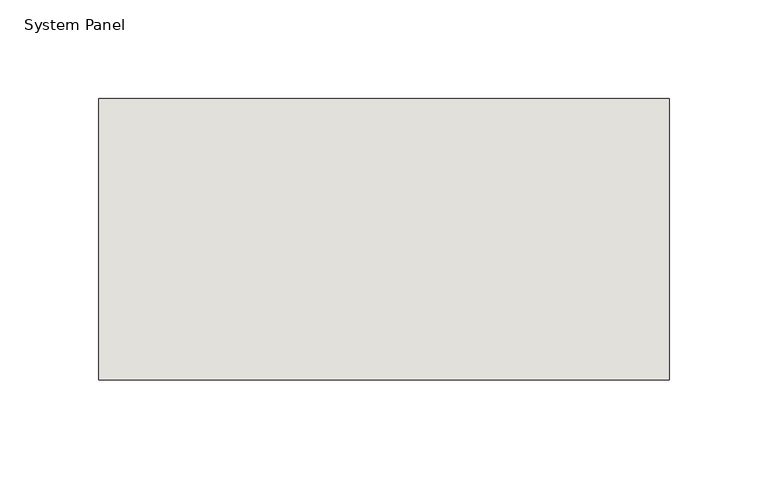
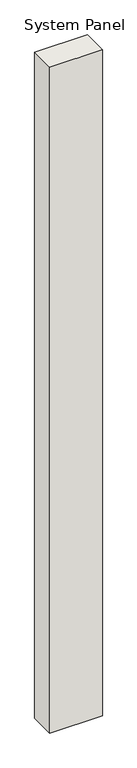
"""IFC4 building model written with IfcOpenShell, lengths in millimetres: wall geometry, System Panel : NLRS_21_CWP_hsb-vulling minerale wol 142 _gen_rsf."""

from ifc_helpers import new_model, si_unit, origin, origin_with_axes, place, context, project, spatial, polyline, outline, extrude, source, transform, mapped, element, save


def system_panel_3da1e079(model_context):
    return source(origin(), model_context, "Body", "SweptSolid", [
        extrude(outline(polyline([(144.0000002, -71.0), (-144.0000002, -71.0), (-144.0000002, 71.0), (144.0000002, 71.0), (144.0000002, -71.0)])), origin_with_axes(), (0.0, 0.0, 1.0), 3849.0),
    ])


if __name__ == "__main__":
    model = new_model("IFC4")
    model_context = context("Model", 3, world=origin())
    ifc_project = project(units=[si_unit("LENGTHUNIT", "METRE", prefix="MILLI")], contexts=[model_context])
    site = spatial("IfcSite", under=ifc_project)
    building = spatial("IfcBuilding", under=site)
    placement = place(None, origin())
    system_panel_shape = system_panel_3da1e079(model_context)
    element("IfcWall", 1, ObjectType="System Panel : NLRS_21_CWP_hsb-vulling minerale wol 142 _gen_rsf", at=placement, inside=building, context=model_context, shape_type="MappedRepresentation", body=[
        mapped(system_panel_shape, transform((0.0, 0.0, 0.0), x_axis=(1.0, 0.0, 0.0), y_axis=(0.0, 1.0, 0.0), z_axis=(0.0, 0.0, 1.0))),
    ])
    save(model, "model.ifc")

# Revit data of these elements
# Type "System Panel : NLRS_21_CWP_hsb-vulling minerale wol 142 _gen_rsf"
#   Type IfcGUID = "07M7mRoiH1CR8m_RSKIwpC"
#   Assembly Code = "21.23"
#   IfcExportAs = "IfcWall"
# Element 1 (IfcWall, "System Panel : NLRS_21_CWP_hsb-vulling minerale wol 142 _gen_rsf")
#   Materials on its faces: "NLRS_m1_isolatie minerale wol_gen_rsf"
# Materials
#   "NLRS_m1_isolatie minerale wol_gen_rsf": class "M - Anorganische materialen", colour RGB 200 200 140, transparency 0, Keynote = "m1", Manufacturer = "Revit Standards Foundation", URL = "www.revitstandards.org", Description = "isolatie minerale wol", Cost = 0
